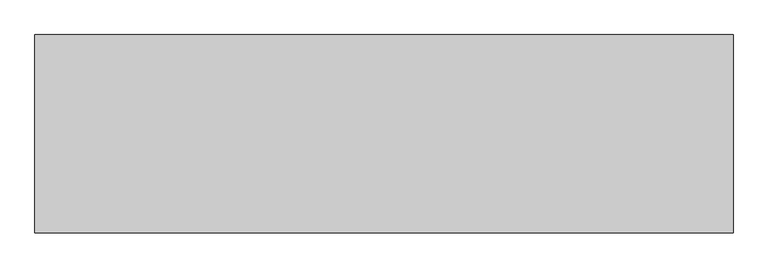
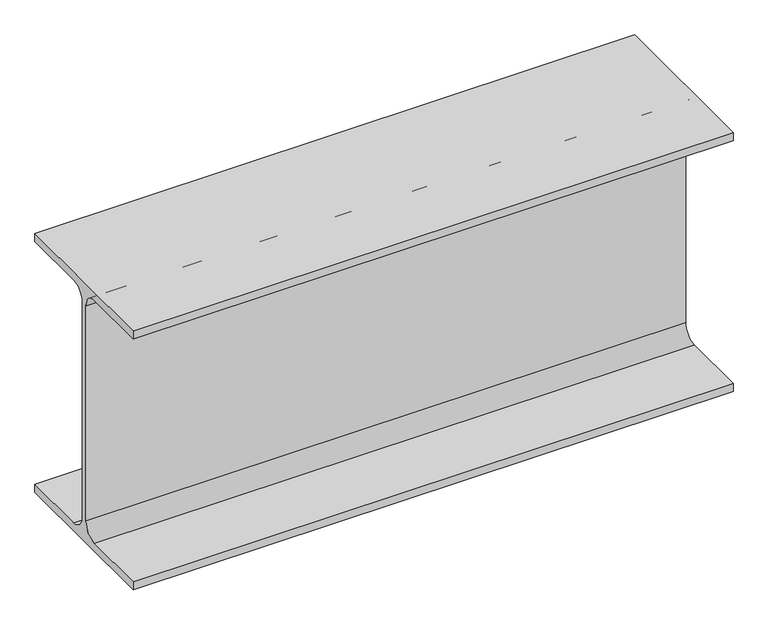
"""IFC4 building model written with IfcOpenShell, lengths in millimetres: beam geometry, 0912_Steel Framing_H-KSD3502 : H_SB_ASB_H-482x300x11x15."""

from ifc_helpers import new_model, si_unit, point, frame, frame_2d, origin, place, context, project, spatial, polyline, circle_curve, trimmed, segment, composite_curve, outline, extrude, source, transform, mapped, element, save


def beam_c6d39c45(model_context):
    return source(origin(), model_context, "Body", "SweptSolid", [
        extrude(outline(composite_curve([segment(polyline([(150.0, -226.0), (150.0, -241.0), (-150.0, -241.0), (-150.0, -226.0), (-31.5, -226.0)]), True, "CONTINUOUS"), segment(trimmed(circle_curve(frame_2d((-31.5, -200.0)), 26.0), [point((-31.5, -226.0))], [point((-5.5, -200.0))], True, "CARTESIAN"), True, "CONTINUOUS"), segment(polyline([(-5.5, -200.0), (-5.5, 200.0)]), True, "CONTINUOUS"), segment(trimmed(circle_curve(frame_2d((-31.5, 200.0)), 26.0), [point((-5.5, 200.0))], [point((-31.5, 226.0))], True, "CARTESIAN"), True, "CONTINUOUS"), segment(polyline([(-31.5, 226.0), (-150.0, 226.0), (-150.0, 241.0), (150.0, 241.0), (150.0, 226.0), (31.5, 226.0)]), True, "CONTINUOUS"), segment(trimmed(circle_curve(frame_2d((31.5, 200.0)), 26.0), [point((31.5, 226.0))], [point((5.5, 200.0))], True, "CARTESIAN"), True, "CONTINUOUS"), segment(polyline([(5.5, 200.0), (5.5, -200.0)]), True, "CONTINUOUS"), segment(trimmed(circle_curve(frame_2d((31.5, -200.0)), 26.0), [point((5.5, -200.0))], [point((31.5, -226.0))], True, "CARTESIAN"), True, "CONTINUOUS"), segment(polyline([(31.5, -226.0), (150.0, -226.0)]), True, "CONTINUOUS")], self_intersect=False)), frame((-527.8, 0.0, 0.0), z_axis=(1.0, 0.0, 0.0), x_axis=(0.0, 1.0, 0.0)), (0.0, 0.0, 1.0), 1055.6),
    ])


if __name__ == "__main__":
    model = new_model("IFC4")
    model_context = context("Model", 3, world=origin())
    ifc_project = project(units=[si_unit("LENGTHUNIT", "METRE", prefix="MILLI")], contexts=[model_context])
    site = spatial("IfcSite", under=ifc_project)
    building = spatial("IfcBuilding", under=site)
    placement = place(None, origin())
    beam_shape = beam_c6d39c45(model_context)
    element("IfcBeam", 1, ObjectType="0912_Steel Framing_H-KSD3502 : H_SB_ASB_H-482x300x11x15", at=placement, inside=building, context=model_context, shape_type="MappedRepresentation", body=[
        mapped(beam_shape, transform((0.0, 0.0, 0.0), x_axis=(1.0, 0.0, 0.0), y_axis=(0.0, 1.0, 0.0), z_axis=(0.0, 0.0, 1.0))),
    ])
    save(model, "model.ifc")

# Revit data of these elements
# Type "0912_Steel Framing_H-KSD3502 : H_SB_ASB_H-482x300x11x15"
#   H_WM Code_1 = "S01AA001-00001 | Main Steel Structure Fabrication Work | Shelter/Building | Heavy Steel - Standard (Weight≥90KG/M) | Material: (   )"
#   H_WM Code_2 = "S03AA027-00001 | Main Steel Structure Erection Work | Shelter/Building | Heavy Steel (Weight≥90KG/M) | Material: (   )"
#   H_WM Code_3 = "S01AA010-00001 | Main Steel Structure Fabrication Work | Shelter/Building | Steel Painting/Coating | for Non-Fireproofed Steel Surface, Surface Preparation, Primer, Second & Final Coat | Material: (   )"
#   H_Q'ty Cal Type Tag = "SB-Q2"
#   Width = 30.0 cm
#   Web Thickness = 1.1 cm
#   Web Fillet = 2.6 cm
#   Warping Constant = 3680000.0 cm⁶
#   W = 0
#   Torsional Moment of Inertia = 88.2192 cm⁴
#   Section Area = 145.5 cm²
#   Plastic Modulus weak axis = 695.0 cm³
#   Plastic Modulus strong axis = 2790.0 cm³
#   Perimeter = 2.10 m²/m
#   Nominal Weight = 114.00 kgf/m
#   Moment of Inertia weak axis = 6760.00 cm⁴
#   Moment of Inertia strong axis = 60400.00 cm⁴
#   Height = 48.2 cm
#   Flange Thickness = 1.5 cm
#   Elastic Modulus weak axis = 451.0 cm³
#   Elastic Modulus strong axis = 2500.0 cm³
#   Centroid Vertical = 24.1 cm
#   Centroid Horizontal = 15.0 cm
#   Ix = 604000000
#   Length [instance default] = 1.5240 m
#   Zx = 2790000
#   b = 0.3000 m
#   h = 0.4820 m
#   r = 0.0260 m
#   s = 0.0110 m
#   t = 0.0150 m
#   A = 0.01455 m²
#   Structural Material [instance default] = Steel, 45-345
#   Assembly Code = ""
# Element 1 (IfcBeam, "0912_Steel Framing_H-KSD3502 : H_SB_ASB_H-482x300x11x15")
#   Structural Material = none
# Materials
#   "Steel, 45-345": class "Metal", colour RGB 189 187 185, transparency 0, Description = "Steel 345 MPa", Cost = 0
